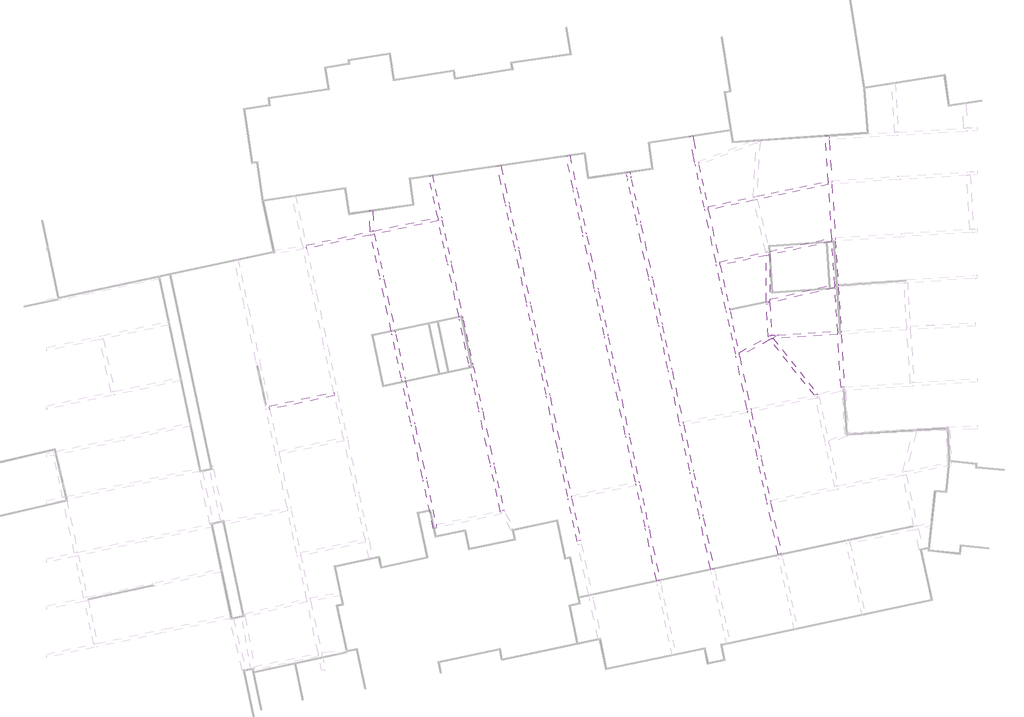
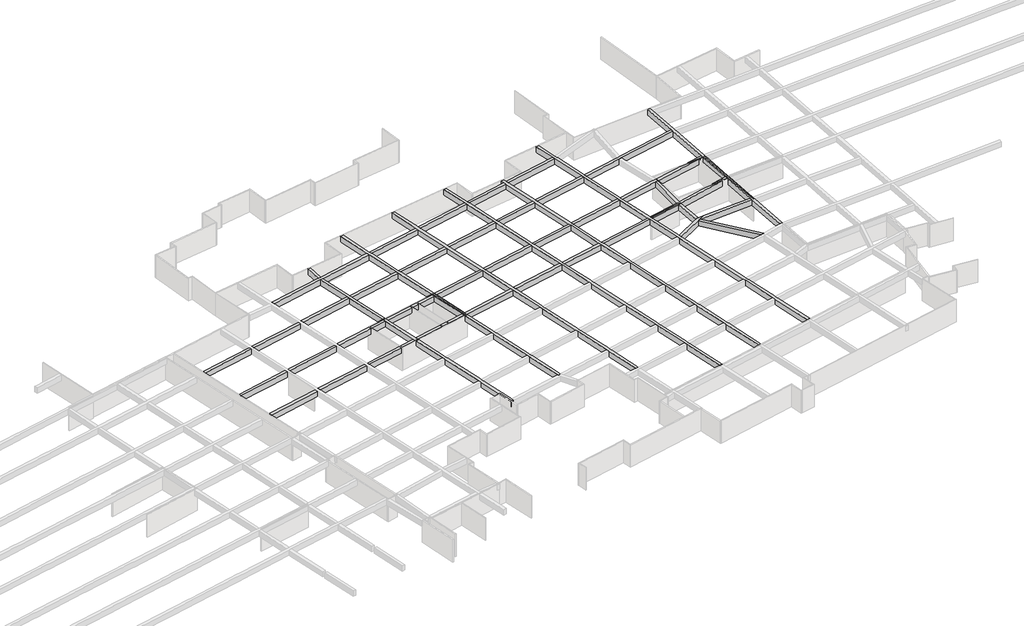
# One storey, part 10 of 14: 18 beams.
"""IFC4 building model written with IfcOpenShell, lengths in millimetres."""

from ifc_helpers import new_model, si_unit, frame, origin, place, context, project, spatial, polyline, outline, extrude, faceted_brep, element, save

model = new_model("IFC4")

# Units and contexts
model_context = context("Model", 3, world=origin())
ifc_project = project(units=[si_unit("LENGTHUNIT", "METRE", prefix="MILLI")], contexts=[model_context])

# Site, building, storey
site = spatial("IfcSite", under=ifc_project)
building = spatial("IfcBuilding", under=site)
storey = spatial("IfcBuildingStorey", under=building, Name="户型图", Elevation=0.0)

# Beams
placement = place(None, origin())
element("IfcBeam", 1, ObjectType="混凝土 - 矩形梁 : KL_beam", at=placement, inside=storey, context=model_context, shape_type="SweptSolid", body=[
    extrude(outline(polyline([(-247291.3597024, -139083.8420876), (-246891.9078885, -139062.9077051), (-246769.3406579, -141401.6297867), (-247165.4767913, -141485.8311212), (-247291.3597024, -139083.8420876)])), frame((0.0, 0.0, 2500.0), z_axis=(0.0, 0.0, 1.0), x_axis=(1.0, 0.0, 0.0)), (0.0, 0.0, 1.0), 800.0),
])
element("IfcBeam", 2, ObjectType="混凝土 - 矩形梁 : KL_beam", at=placement, inside=storey, context=model_context, shape_type="Brep", body=[
    faceted_brep([(-239502.5663622, -175696.1273321, 3300.0), (-239502.5663622, -175696.1273321, 2500.0), (-239585.7310386, -175304.8682918, 2500.0), (-240656.2680649, -170268.3875645, 2500.0), (-240739.4335016, -169877.124947, 2500.0), (-242007.8205291, -163909.833147, 2500.0), (-242090.9852054, -163518.5741067, 2500.0), (-243116.5813419, -158693.5236429, 2500.0), (-243199.7460182, -158302.2646026, 2500.0), (-244253.2667899, -153345.839059, 2500.0), (-244336.4314662, -152954.5800187, 2500.0), (-245612.0065383, -146953.4711277, 2500.0), (-245695.1712146, -146562.2120874, 2500.0), (-246707.9389128, -141797.5146808, 2500.0), (-246707.9389128, -141797.5146808, 3300.0), (-245695.1712146, -146562.2120874, 3300.0), (-245612.0065383, -146953.4711277, 3300.0), (-244336.4314662, -152954.5800187, 3300.0), (-244253.2667899, -153345.839059, 3300.0), (-243199.7460182, -158302.2646026, 3300.0), (-243116.5813419, -158693.5236429, 3300.0), (-242090.9852054, -163518.5741067, 3300.0), (-242007.8205291, -163909.833147, 3300.0), (-240739.4335016, -169877.124947, 3300.0), (-240656.2680649, -170268.3875645, 3300.0), (-239585.7310386, -175304.8682918, 3300.0), (-247099.1979531, -141880.6793572, 2500.0), (-247099.1979531, -141880.6793572, 3300.0), (-246086.4302549, -146645.3767637, 3300.0), (-246003.2655786, -147036.635804, 3300.0), (-244727.6905065, -153037.7446951, 3300.0), (-244644.5258302, -153429.0037354, 3300.0), (-243591.0050585, -158385.4292789, 3300.0), (-243507.8403822, -158776.6883192, 3300.0), (-242482.2442457, -163601.738783, 3300.0), (-242399.0795694, -163992.9978233, 3300.0), (-241130.3369189, -169961.9626978, 3300.0), (-241047.1714822, -170353.2253152, 3300.0), (-239893.8254025, -175779.2920084, 3300.0), (-246086.4302549, -146645.3767637, 2500.0), (-246003.2655786, -147036.635804, 2500.0), (-244727.6905065, -153037.7446951, 2500.0), (-244644.5258302, -153429.0037354, 2500.0), (-243591.0050585, -158385.4292789, 2500.0), (-243507.8403822, -158776.6883192, 2500.0), (-242482.2442457, -163601.738783, 2500.0), (-242399.0795694, -163992.9978233, 2500.0), (-241130.3369189, -169961.9626978, 2500.0), (-241047.1714822, -170353.2253152, 2500.0), (-239893.8254025, -175779.2920084, 2500.0)], [[[0, 1, 2, 3, 4, 5, 6, 7, 8, 9, 10, 11, 12, 13, 14, 15, 16, 17, 18, 19, 20, 21, 22, 23, 24, 25]], [[14, 13, 26, 27]], [[14, 27, 28, 29, 30, 31, 32, 33, 34, 35, 36, 37, 38, 0, 25, 24, 23, 22, 21, 20, 19, 18, 17, 16, 15]], [[27, 26, 39, 40, 41, 42, 43, 44, 45, 46, 47, 48, 49, 38, 37, 36, 35, 34, 33, 32, 31, 30, 29, 28]], [[26, 13, 12, 11, 10, 9, 8, 7, 6, 5, 4, 3, 2, 1, 49, 48, 47, 46, 45, 44, 43, 42, 41, 40, 39]], [[0, 38, 49, 1]]]),
])
element("IfcBeam", 3, ObjectType="混凝土 - 矩形梁 : KL_beam", at=placement, inside=storey, context=model_context, shape_type="Brep", body=[
    faceted_brep([(-240003.3061587, -134987.1905484, 3300.0), (-240003.3061587, -134987.1905484, 2500.0), (-240394.565199, -135070.3552247, 2500.0), (-240394.565199, -135070.3552247, 3300.0), (-232154.5574648, -173836.5437133, 3300.0), (-231776.7079802, -173690.2920379, 3300.0), (-231785.9170748, -173646.966654, 3300.0), (-232863.5435036, -168577.1329101, 3300.0), (-232946.7089403, -168185.8702927, 3300.0), (-234208.0065653, -162251.9315092, 3300.0), (-234291.1712416, -161860.6724689, 3300.0), (-235316.7673781, -157035.6220051, 3300.0), (-235399.9320544, -156644.3629648, 3300.0), (-236453.4528261, -151687.9374212, 3300.0), (-236536.6175025, -151296.6783809, 3300.0), (-237812.1925745, -145295.5694899, 3300.0), (-237895.3572509, -144904.3104496, 3300.0), (-238908.124949, -140139.613043, 3300.0), (-238991.2896253, -139748.3540027, 3300.0), (-239382.5486656, -139831.5186791, 3300.0), (-239299.3839893, -140222.7777194, 3300.0), (-238286.6162912, -144987.4751259, 3300.0), (-238203.4516148, -145378.7341662, 3300.0), (-236927.8765428, -151379.8430573, 3300.0), (-236844.7118664, -151771.1020976, 3300.0), (-235791.1910947, -156727.5276411, 3300.0), (-235708.0264184, -157118.7866814, 3300.0), (-234682.4302819, -161943.8371452, 3300.0), (-234599.2656056, -162335.0961855, 3300.0), (-233337.6123577, -168270.7080435, 3300.0), (-233254.446921, -168661.9706609, 3300.0), (-232177.1761151, -173730.1313303, 3300.0), (-232154.5574648, -173836.5437133, 2500.0), (-239382.5486656, -139831.5186791, 2500.0), (-239299.3839893, -140222.7777194, 2500.0), (-238286.6162912, -144987.4751259, 2500.0), (-238203.4516148, -145378.7341662, 2500.0), (-236927.8765428, -151379.8430573, 2500.0), (-236844.7118664, -151771.1020976, 2500.0), (-235791.1910947, -156727.5276411, 2500.0), (-235708.0264184, -157118.7866814, 2500.0), (-234682.4302819, -161943.8371452, 2500.0), (-234599.2656056, -162335.0961855, 2500.0), (-233337.6123577, -168270.7080435, 2500.0), (-233254.446921, -168661.9706609, 2500.0), (-232177.1761151, -173730.1313303, 2500.0), (-231776.7079802, -173690.2920379, 2500.0), (-238991.2896253, -139748.3540027, 2500.0), (-238908.124949, -140139.613043, 2500.0), (-237895.3572509, -144904.3104496, 2500.0), (-237812.1925745, -145295.5694899, 2500.0), (-236536.6175025, -151296.6783809, 2500.0), (-236453.4528261, -151687.9374212, 2500.0), (-235399.9320544, -156644.3629648, 2500.0), (-235316.7673781, -157035.6220051, 2500.0), (-234291.1712416, -161860.6724689, 2500.0), (-234208.0065653, -162251.9315092, 2500.0), (-232946.7089403, -168185.8702927, 2500.0), (-232863.5435036, -168577.1329101, 2500.0), (-231785.9170748, -173646.966654, 2500.0)], [[[0, 1, 2, 3]], [[4, 5, 6, 7, 8, 9, 10, 11, 12, 13, 14, 15, 16, 17, 18, 0, 3, 19, 20, 21, 22, 23, 24, 25, 26, 27, 28, 29, 30, 31]], [[32, 4, 31, 30, 29, 28, 27, 26, 25, 24, 23, 22, 21, 20, 19, 3, 2, 33, 34, 35, 36, 37, 38, 39, 40, 41, 42, 43, 44, 45]], [[46, 32, 45, 44, 43, 42, 41, 40, 39, 38, 37, 36, 35, 34, 33, 2, 1, 47, 48, 49, 50, 51, 52, 53, 54, 55, 56, 57, 58, 59]], [[5, 46, 59, 58, 57, 56, 55, 54, 53, 52, 51, 50, 49, 48, 47, 1, 0, 18, 17, 16, 15, 14, 13, 12, 11, 10, 9, 8, 7, 6]], [[5, 4, 32, 46]]]),
])
element("IfcBeam", 4, ObjectType="混凝土 - 矩形梁 : KL_beam", at=placement, inside=storey, context=model_context, shape_type="Brep", body=[
    faceted_brep([(-232107.9736676, -133827.7635984, 3300.0), (-232107.9736676, -133827.7635984, 2500.0), (-232499.2327078, -133910.9282747, 2500.0), (-232499.2327078, -133910.9282747, 3300.0), (-231592.7191403, -138175.7392992, 3300.0), (-231509.554464, -138566.9983395, 3300.0), (-230496.7867659, -143331.695746, 3300.0), (-230413.6220895, -143722.9547863, 3300.0), (-229138.0470174, -149724.0636774, 3300.0), (-229054.8823411, -150115.3227177, 3300.0), (-228001.3615694, -155071.7482612, 3300.0), (-227918.1968931, -155463.0073015, 3300.0), (-226892.6007566, -160288.0577653, 3300.0), (-226809.4360803, -160679.3168056, 3300.0), (-225554.8631598, -166581.6183418, 3300.0), (-225471.6977231, -166972.8809592, 3300.0), (-224387.3465898, -172074.3519504, 3300.0), (-224304.1819135, -172465.6109907, 3300.0), (-223290.3781842, -177235.1825406, 3300.0), (-222899.1191439, -177152.0178643, 3300.0), (-223912.9228732, -172382.4463144, 3300.0), (-223996.0875495, -171991.1872741, 3300.0), (-225080.7943058, -166888.0432085, 3300.0), (-225163.9597425, -166496.7805911, 3300.0), (-226418.17704, -160596.1521293, 3300.0), (-226501.3417163, -160204.893089, 3300.0), (-227526.9378528, -155379.8426252, 3300.0), (-227610.1025291, -154988.5835849, 3300.0), (-228663.6233008, -150032.1580413, 3300.0), (-228746.7879771, -149640.899001, 3300.0), (-230022.3630492, -143639.79011, 3300.0), (-230105.5277256, -143248.5310697, 3300.0), (-231118.2954237, -138483.8336631, 3300.0), (-231201.4601, -138092.5746229, 3300.0), (-231592.7191403, -138175.7392992, 2500.0), (-231509.554464, -138566.9983395, 2500.0), (-230496.7867659, -143331.695746, 2500.0), (-230413.6220895, -143722.9547863, 2500.0), (-229138.0470174, -149724.0636774, 2500.0), (-229054.8823411, -150115.3227177, 2500.0), (-228001.3615694, -155071.7482612, 2500.0), (-227918.1968931, -155463.0073015, 2500.0), (-226892.6007566, -160288.0577653, 2500.0), (-226809.4360803, -160679.3168056, 2500.0), (-225554.8631598, -166581.6183418, 2500.0), (-225471.6977231, -166972.8809592, 2500.0), (-224387.3465898, -172074.3519504, 2500.0), (-224304.1819135, -172465.6109907, 2500.0), (-223290.3781842, -177235.1825406, 2500.0), (-231201.4601, -138092.5746229, 2500.0), (-231118.2954237, -138483.8336631, 2500.0), (-230105.5277256, -143248.5310697, 2500.0), (-230022.3630492, -143639.79011, 2500.0), (-228746.7879771, -149640.899001, 2500.0), (-228663.6233008, -150032.1580413, 2500.0), (-227610.1025291, -154988.5835849, 2500.0), (-227526.9378528, -155379.8426252, 2500.0), (-226501.3417163, -160204.893089, 2500.0), (-226418.17704, -160596.1521293, 2500.0), (-225163.9597425, -166496.7805911, 2500.0), (-225080.7943058, -166888.0432085, 2500.0), (-223996.0875495, -171991.1872741, 2500.0), (-223912.9228732, -172382.4463144, 2500.0), (-222899.1191439, -177152.0178643, 2500.0)], [[[0, 1, 2, 3]], [[0, 3, 4, 5, 6, 7, 8, 9, 10, 11, 12, 13, 14, 15, 16, 17, 18, 19, 20, 21, 22, 23, 24, 25, 26, 27, 28, 29, 30, 31, 32, 33]], [[3, 2, 34, 35, 36, 37, 38, 39, 40, 41, 42, 43, 44, 45, 46, 47, 48, 18, 17, 16, 15, 14, 13, 12, 11, 10, 9, 8, 7, 6, 5, 4]], [[2, 1, 49, 50, 51, 52, 53, 54, 55, 56, 57, 58, 59, 60, 61, 62, 63, 48, 47, 46, 45, 44, 43, 42, 41, 40, 39, 38, 37, 36, 35, 34]], [[1, 0, 33, 32, 31, 30, 29, 28, 27, 26, 25, 24, 23, 22, 21, 20, 19, 63, 62, 61, 60, 59, 58, 57, 56, 55, 54, 53, 52, 51, 50, 49]], [[19, 18, 48, 63]]]),
])
element("IfcBeam", 5, ObjectType="混凝土 - 矩形梁 : KL_beam", at=placement, inside=storey, context=model_context, shape_type="Brep", body=[
    faceted_brep([(-224568.0292654, -132746.4320366, 3300.0), (-224176.7702251, -132663.2673603, 3300.0), (-224176.7702251, -132663.2673603, 2500.0), (-224568.0292654, -132746.4320366, 2500.0), (-223767.5383344, -136512.4457726, 3300.0), (-223684.3736581, -136903.7048129, 3300.0), (-222671.60596, -141668.4022195, 3300.0), (-222588.4412837, -142059.6612598, 3300.0), (-221312.8662116, -148060.7701508, 3300.0), (-221229.7015352, -148452.0291911, 3300.0), (-220176.1807635, -153408.4547347, 3300.0), (-220093.0160872, -153799.713775, 3300.0), (-219067.4199507, -158624.7642388, 3300.0), (-218984.2552744, -159016.023279, 3300.0), (-217736.7948129, -164884.8633268, 3300.0), (-217653.6293762, -165276.1259443, 3300.0), (-216562.1657839, -170411.0584239, 3300.0), (-216479.0011076, -170802.3174642, 3300.0), (-215465.1973783, -175571.8890141, 3300.0), (-215382.032702, -175963.1480544, 3300.0), (-214134.7118605, -181831.3312414, 3300.0), (-213743.4528202, -181748.166565, 3300.0), (-214990.7736617, -175879.9833781, 3300.0), (-215073.938338, -175488.7243378, 3300.0), (-216087.7420673, -170719.1527879, 3300.0), (-216170.9067436, -170327.8937476, 3300.0), (-217262.7259588, -165191.2881935, 3300.0), (-217345.8913955, -164800.0255761, 3300.0), (-218592.9962341, -158932.8586027, 3300.0), (-218676.1609104, -158541.5995624, 3300.0), (-219701.7570469, -153716.5490987, 3300.0), (-219784.9217232, -153325.2900584, 3300.0), (-220838.4424949, -148368.8645148, 3300.0), (-220921.6071713, -147977.6054745, 3300.0), (-222197.1822434, -141976.4965835, 3300.0), (-222280.3469197, -141585.2375432, 3300.0), (-223293.1146178, -136820.5401366, 3300.0), (-223376.2792942, -136429.2810963, 3300.0), (-213743.4528202, -181748.166565, 2500.0), (-214990.7736617, -175879.9833781, 2500.0), (-215073.938338, -175488.7243378, 2500.0), (-216087.7420673, -170719.1527879, 2500.0), (-216170.9067436, -170327.8937476, 2500.0), (-217262.7259588, -165191.2881935, 2500.0), (-217345.8913955, -164800.0255761, 2500.0), (-218592.9962341, -158932.8586027, 2500.0), (-218676.1609104, -158541.5995624, 2500.0), (-219701.7570469, -153716.5490987, 2500.0), (-219784.9217232, -153325.2900584, 2500.0), (-220838.4424949, -148368.8645148, 2500.0), (-220921.6071713, -147977.6054745, 2500.0), (-222197.1822434, -141976.4965835, 2500.0), (-222280.3469197, -141585.2375432, 2500.0), (-223293.1146178, -136820.5401366, 2500.0), (-223376.2792942, -136429.2810963, 2500.0), (-214134.7118605, -181831.3312414, 2500.0), (-215382.032702, -175963.1480544, 2500.0), (-215465.1973783, -175571.8890141, 2500.0), (-216479.0011076, -170802.3174642, 2500.0), (-216562.1657839, -170411.0584239, 2500.0), (-217653.6293762, -165276.1259443, 2500.0), (-217736.7948129, -164884.8633268, 2500.0), (-218984.2552744, -159016.023279, 2500.0), (-219067.4199507, -158624.7642388, 2500.0), (-220093.0160872, -153799.713775, 2500.0), (-220176.1807635, -153408.4547347, 2500.0), (-221229.7015352, -148452.0291911, 2500.0), (-221312.8662116, -148060.7701508, 2500.0), (-222588.4412837, -142059.6612598, 2500.0), (-222671.60596, -141668.4022195, 2500.0), (-223684.3736581, -136903.7048129, 2500.0), (-223767.5383344, -136512.4457726, 2500.0)], [[[0, 1, 2, 3]], [[1, 0, 4, 5, 6, 7, 8, 9, 10, 11, 12, 13, 14, 15, 16, 17, 18, 19, 20, 21, 22, 23, 24, 25, 26, 27, 28, 29, 30, 31, 32, 33, 34, 35, 36, 37]], [[2, 1, 37, 36, 35, 34, 33, 32, 31, 30, 29, 28, 27, 26, 25, 24, 23, 22, 21, 38, 39, 40, 41, 42, 43, 44, 45, 46, 47, 48, 49, 50, 51, 52, 53, 54]], [[3, 2, 54, 53, 52, 51, 50, 49, 48, 47, 46, 45, 44, 43, 42, 41, 40, 39, 38, 55, 56, 57, 58, 59, 60, 61, 62, 63, 64, 65, 66, 67, 68, 69, 70, 71]], [[0, 3, 71, 70, 69, 68, 67, 66, 65, 64, 63, 62, 61, 60, 59, 58, 57, 56, 55, 20, 19, 18, 17, 16, 15, 14, 13, 12, 11, 10, 9, 8, 7, 6, 5, 4]], [[20, 55, 38, 21]]]),
])
element("IfcBeam", 6, ObjectType="混凝土 - 矩形梁 : KL_beam", at=placement, inside=storey, context=model_context, shape_type="Brep", body=[
    faceted_brep([(-217241.693878, -134575.5020687, 3300.0), (-217241.693878, -134575.5020687, 2500.0), (-217632.9529183, -134658.666745, 2500.0), (-217632.9529183, -134658.666745, 3300.0), (-207888.3079023, -180503.6170932, 3300.0), (-207497.048862, -180420.4524169, 3300.0), (-208744.3697035, -174552.2692299, 3300.0), (-208827.5343798, -174161.0101896, 3300.0), (-209841.3381091, -169391.4386397, 3300.0), (-209924.5027854, -169000.1795994, 3300.0), (-211021.0898908, -163841.1428861, 3300.0), (-211104.2672354, -163449.824246, 3300.0), (-212346.5922759, -157605.1444546, 3300.0), (-212429.7569523, -157213.8854143, 3300.0), (-213455.3530887, -152388.8349505, 3300.0), (-213538.5177651, -151997.5759102, 3300.0), (-214592.0385368, -147041.1503666, 3300.0), (-214675.2032131, -146649.8913263, 3300.0), (-215950.7782852, -140648.7824353, 3300.0), (-216033.9429615, -140257.523395, 3300.0), (-217046.7106596, -135492.8259885, 3300.0), (-217129.875336, -135101.5669482, 3300.0), (-217521.1343763, -135184.7316245, 3300.0), (-217437.9696999, -135575.9906648, 3300.0), (-216425.2020018, -140340.6880713, 3300.0), (-216342.0373255, -140731.9471116, 3300.0), (-215066.4622534, -146733.0560027, 3300.0), (-214983.2975771, -147124.315043, 3300.0), (-213929.7768053, -152080.7405865, 3300.0), (-213846.612129, -152471.9996268, 3300.0), (-212821.0159926, -157297.0500906, 3300.0), (-212737.8513162, -157688.3091309, 3300.0), (-211496.0683326, -163530.4387449, 3300.0), (-211412.902896, -163921.7013623, 3300.0), (-210315.7618257, -169083.3442757, 3300.0), (-210232.5971494, -169474.603316, 3300.0), (-209218.7934201, -174244.1748659, 3300.0), (-209135.6287438, -174635.4339062, 3300.0), (-207888.3079023, -180503.6170932, 2500.0), (-217521.1343763, -135184.7316245, 2500.0), (-217437.9696999, -135575.9906648, 2500.0), (-216425.2020018, -140340.6880713, 2500.0), (-216342.0373255, -140731.9471116, 2500.0), (-215066.4622534, -146733.0560027, 2500.0), (-214983.2975771, -147124.315043, 2500.0), (-213929.7768053, -152080.7405865, 2500.0), (-213846.612129, -152471.9996268, 2500.0), (-212821.0159926, -157297.0500906, 2500.0), (-212737.8513162, -157688.3091309, 2500.0), (-211496.0683326, -163530.4387449, 2500.0), (-211412.902896, -163921.7013623, 2500.0), (-210315.7618257, -169083.3442757, 2500.0), (-210232.5971494, -169474.603316, 2500.0), (-209218.7934201, -174244.1748659, 2500.0), (-209135.6287438, -174635.4339062, 2500.0), (-207497.048862, -180420.4524169, 2500.0), (-217129.875336, -135101.5669482, 2500.0), (-217046.7106596, -135492.8259885, 2500.0), (-216033.9429615, -140257.523395, 2500.0), (-215950.7782852, -140648.7824353, 2500.0), (-214675.2032131, -146649.8913263, 2500.0), (-214592.0385368, -147041.1503666, 2500.0), (-213538.5177651, -151997.5759102, 2500.0), (-213455.3530887, -152388.8349505, 2500.0), (-212429.7569523, -157213.8854143, 2500.0), (-212346.5922759, -157605.1444546, 2500.0), (-211104.2672354, -163449.824246, 2500.0), (-211021.0898908, -163841.1428861, 2500.0), (-209924.5027854, -169000.1795994, 2500.0), (-209841.3381091, -169391.4386397, 2500.0), (-208827.5343798, -174161.0101896, 2500.0), (-208744.3697035, -174552.2692299, 2500.0)], [[[0, 1, 2, 3]], [[4, 5, 6, 7, 8, 9, 10, 11, 12, 13, 14, 15, 16, 17, 18, 19, 20, 21, 0, 3, 22, 23, 24, 25, 26, 27, 28, 29, 30, 31, 32, 33, 34, 35, 36, 37]], [[38, 4, 37, 36, 35, 34, 33, 32, 31, 30, 29, 28, 27, 26, 25, 24, 23, 22, 3, 2, 39, 40, 41, 42, 43, 44, 45, 46, 47, 48, 49, 50, 51, 52, 53, 54]], [[55, 38, 54, 53, 52, 51, 50, 49, 48, 47, 46, 45, 44, 43, 42, 41, 40, 39, 2, 1, 56, 57, 58, 59, 60, 61, 62, 63, 64, 65, 66, 67, 68, 69, 70, 71]], [[5, 55, 71, 70, 69, 68, 67, 66, 65, 64, 63, 62, 61, 60, 59, 58, 57, 56, 1, 0, 21, 20, 19, 18, 17, 16, 15, 14, 13, 12, 11, 10, 9, 8, 7, 6]], [[5, 4, 38, 55]]]),
])
element("IfcBeam", 7, ObjectType="混凝土 - 矩形梁 : KL_beam", at=placement, inside=storey, context=model_context, shape_type="Brep", body=[
    faceted_brep([(-210361.4643641, -130516.7008137, 3300.0), (-209970.2053238, -130433.5361374, 3300.0), (-209970.2053238, -130433.5361374, 2500.0), (-210361.4643641, -130516.7008137, 2500.0), (-209721.6277704, -133526.8953176, 3300.0), (-209638.463094, -133918.1543579, 3300.0), (-208625.6953959, -138682.8517645, 3300.0), (-208542.5307196, -139074.1108048, 3300.0), (-207266.9556475, -145075.2196958, 3300.0), (-207183.7909711, -145466.4787361, 3300.0), (-206130.2701994, -150422.9042797, 3300.0), (-206047.1055231, -150814.16332, 3300.0), (-205021.5093866, -155639.2137837, 3300.0), (-204938.3447103, -156030.472824, 3300.0), (-203668.5336742, -162004.4640578, 3300.0), (-203585.3563296, -162395.7826978, 3300.0), (-202516.2552198, -167425.5079689, 3300.0), (-202433.0905435, -167816.7670092, 3300.0), (-201419.2868142, -172586.3385591, 3300.0), (-201336.1221379, -172977.5975994, 3300.0), (-200110.5246312, -178743.5805315, 3300.0), (-199719.2655909, -178660.4158551, 3300.0), (-200944.8630976, -172894.432923, 3300.0), (-201028.0277739, -172503.1738827, 3300.0), (-202041.8315032, -167733.6023328, 3300.0), (-202124.9961795, -167342.3432925, 3300.0), (-203193.377801, -162316.0029476, 3300.0), (-203276.5424774, -161924.7439073, 3300.0), (-204557.8986965, -155896.4368576, 3300.0), (-204644.863313, -155487.3005045, 3300.0), (-205655.8464828, -150730.9986436, 3300.0), (-205739.0111591, -150339.7396033, 3300.0), (-206792.5319309, -145383.3140598, 3300.0), (-206875.6966072, -144992.0550195, 3300.0), (-208151.2716793, -138990.9461284, 3300.0), (-208234.4363556, -138599.6870881, 3300.0), (-209253.2346635, -133806.6178935, 3300.0), (-209337.422307, -133410.5461707, 3300.0), (-199719.2655909, -178660.4158551, 2500.0), (-200944.8630976, -172894.432923, 2500.0), (-201028.0277739, -172503.1738827, 2500.0), (-202041.8315032, -167733.6023328, 2500.0), (-202124.9961795, -167342.3432925, 2500.0), (-203193.377801, -162316.0029476, 2500.0), (-203276.5424774, -161924.7439073, 2500.0), (-204557.8986965, -155896.4368576, 2500.0), (-204644.863313, -155487.3005045, 2500.0), (-205655.8464828, -150730.9986436, 2500.0), (-205739.0111591, -150339.7396033, 2500.0), (-206792.5319309, -145383.3140598, 2500.0), (-206875.6966072, -144992.0550195, 2500.0), (-208151.2716793, -138990.9461284, 2500.0), (-208234.4363556, -138599.6870881, 2500.0), (-209253.2346635, -133806.6178935, 2500.0), (-209337.422307, -133410.5461707, 2500.0), (-200110.5246312, -178743.5805315, 2500.0), (-201336.1221379, -172977.5975994, 2500.0), (-201419.2868142, -172586.3385591, 2500.0), (-202433.0905435, -167816.7670092, 2500.0), (-202516.2552198, -167425.5079689, 2500.0), (-203585.3563296, -162395.7826978, 2500.0), (-203668.5336742, -162004.4640578, 2500.0), (-204938.3447103, -156030.472824, 2500.0), (-205021.5093866, -155639.2137837, 2500.0), (-206047.1055231, -150814.16332, 2500.0), (-206130.2701994, -150422.9042797, 2500.0), (-207183.7909711, -145466.4787361, 2500.0), (-207266.9556475, -145075.2196958, 2500.0), (-208542.5307196, -139074.1108048, 2500.0), (-208625.6953959, -138682.8517645, 2500.0), (-209638.463094, -133918.1543579, 2500.0), (-209721.6277704, -133526.8953176, 2500.0)], [[[0, 1, 2, 3]], [[1, 0, 4, 5, 6, 7, 8, 9, 10, 11, 12, 13, 14, 15, 16, 17, 18, 19, 20, 21, 22, 23, 24, 25, 26, 27, 28, 29, 30, 31, 32, 33, 34, 35, 36, 37]], [[2, 1, 37, 36, 35, 34, 33, 32, 31, 30, 29, 28, 27, 26, 25, 24, 23, 22, 21, 38, 39, 40, 41, 42, 43, 44, 45, 46, 47, 48, 49, 50, 51, 52, 53, 54]], [[3, 2, 54, 53, 52, 51, 50, 49, 48, 47, 46, 45, 44, 43, 42, 41, 40, 39, 38, 55, 56, 57, 58, 59, 60, 61, 62, 63, 64, 65, 66, 67, 68, 69, 70, 71]], [[0, 3, 71, 70, 69, 68, 67, 66, 65, 64, 63, 62, 61, 60, 59, 58, 57, 56, 55, 20, 19, 18, 17, 16, 15, 14, 13, 12, 11, 10, 9, 8, 7, 6, 5, 4]], [[20, 55, 38, 21]]]),
])
element("IfcBeam", 8, ObjectType="混凝土 - 矩形梁 : KL_beam", at=placement, inside=storey, context=model_context, shape_type="Brep", body=[
    faceted_brep([(-201469.3690271, -149705.3712489, 3300.0), (-201069.3690271, -149705.3712489, 3300.0), (-201069.3690271, -149294.7612479, 3300.0), (-201069.3690271, -144166.8182311, 3300.0), (-201469.3690271, -144251.8408557, 3300.0), (-201469.3690271, -149432.1991522, 3300.0), (-201469.3690271, -149705.3712489, 2500.0), (-201469.3690271, -144251.8408557, 2500.0), (-201469.3690271, -149432.1991522, 2500.0), (-201069.3690271, -149705.3712489, 2500.0), (-201069.3690271, -144166.8182311, 2500.0), (-201069.3690271, -149294.7612479, 2500.0)], [[[0, 1, 2, 3, 4, 5]], [[6, 0, 5, 4, 7, 8]], [[9, 6, 8, 7, 10, 11]], [[1, 9, 11, 10, 3, 2]], [[1, 0, 6, 9]], [[3, 10, 7, 4]]]),
])
element("IfcBeam", 9, ObjectType="混凝土 - 矩形梁 : KL_beam", at=placement, inside=storey, context=model_context, shape_type="Brep", body=[
    faceted_brep([(-269185.8351032, -151555.3068349, 3300.0), (-269185.8351032, -151555.3068349, 2500.0), (-269102.6704268, -151946.5658752, 2500.0), (-269102.6704268, -151946.5658752, 3300.0), (-261736.5979738, -149971.9226036, 3300.0), (-261653.4332975, -150363.1816439, 3300.0), (-261653.4332975, -150363.1816439, 2500.0), (-261736.5979738, -149971.9226036, 2500.0)], [[[0, 1, 2, 3]], [[4, 5, 6, 7]], [[0, 3, 5, 4]], [[3, 2, 6, 5]], [[2, 1, 7, 6]], [[1, 0, 4, 7]]]),
    faceted_brep([(-208234.4363556, -138599.6870881, 3300.0), (-208151.2716793, -138990.9461284, 3300.0), (-202914.7402599, -137877.8870148, 3300.0), (-202523.4216199, -137794.7096702, 3300.0), (-194295.6524967, -136045.8433552, 3300.0), (-194320.579007, -135642.2054105, 3300.0), (-202549.7970747, -137391.3797083, 3300.0), (-202955.2359711, -137477.558406, 3300.0), (-208151.2716793, -138990.9461284, 2500.0), (-202914.7402599, -137877.8870148, 2500.0), (-202523.4216199, -137794.7096702, 2500.0), (-194295.6524967, -136045.8433552, 2500.0), (-208234.4363556, -138599.6870881, 2500.0), (-202955.2359711, -137477.558406, 2500.0), (-202549.7970747, -137391.3797083, 2500.0), (-194320.579007, -135642.2054105, 2500.0)], [[[0, 1, 2, 3, 4, 5, 6, 7]], [[1, 8, 9, 10, 11, 4, 3, 2]], [[8, 12, 13, 14, 15, 11, 10, 9]], [[12, 0, 7, 6, 5, 15, 14, 13]], [[1, 0, 12, 8]], [[5, 4, 11, 15]]]),
    faceted_brep([(-261262.1742572, -150280.0169676, 3300.0), (-261345.3389335, -149888.7579273, 3300.0), (-261345.3389335, -149888.7579273, 2500.0), (-261262.1742572, -150280.0169676, 2500.0), (-253874.8161124, -148300.8492826, 3300.0), (-253791.6514361, -148692.1083228, 3300.0), (-253791.6514361, -148692.1083228, 2500.0), (-253874.8161124, -148300.8492826, 2500.0)], [[[0, 1, 2, 3]], [[4, 5, 6, 7]], [[1, 0, 5, 4]], [[0, 3, 6, 5]], [[3, 2, 7, 6]], [[2, 1, 4, 7]]]),
    faceted_brep([(-253400.3923958, -148608.9436465, 3300.0), (-253483.5570721, -148217.6846062, 3300.0), (-253483.5570721, -148217.6846062, 2500.0), (-253400.3923958, -148608.9436465, 2500.0), (-246086.4302549, -146645.3767637, 3300.0), (-246003.2655786, -147036.635804, 3300.0), (-246003.2655786, -147036.635804, 2500.0), (-246086.4302549, -146645.3767637, 2500.0)], [[[0, 1, 2, 3]], [[4, 5, 6, 7]], [[1, 0, 5, 4]], [[0, 3, 6, 5]], [[3, 2, 7, 6]], [[2, 1, 4, 7]]]),
    faceted_brep([(-245612.0065383, -146953.4711277, 3300.0), (-245695.1712146, -146562.2120874, 3300.0), (-245695.1712146, -146562.2120874, 2500.0), (-245612.0065383, -146953.4711277, 2500.0), (-238286.6162912, -144987.4751259, 3300.0), (-238203.4516148, -145378.7341662, 3300.0), (-238203.4516148, -145378.7341662, 2500.0), (-238286.6162912, -144987.4751259, 2500.0)], [[[0, 1, 2, 3]], [[4, 5, 6, 7]], [[1, 0, 5, 4]], [[0, 3, 6, 5]], [[3, 2, 7, 6]], [[2, 1, 4, 7]]]),
    faceted_brep([(-237812.1925745, -145295.5694899, 3300.0), (-237895.3572509, -144904.3104496, 3300.0), (-237895.3572509, -144904.3104496, 2500.0), (-237812.1925745, -145295.5694899, 2500.0), (-230496.7867659, -143331.695746, 3300.0), (-230413.6220895, -143722.9547863, 3300.0), (-230413.6220895, -143722.9547863, 2500.0), (-230496.7867659, -143331.695746, 2500.0)], [[[0, 1, 2, 3]], [[4, 5, 6, 7]], [[1, 0, 5, 4]], [[0, 3, 6, 5]], [[3, 2, 7, 6]], [[2, 1, 4, 7]]]),
    faceted_brep([(-230022.3630492, -143639.79011, 3300.0), (-230105.5277256, -143248.5310697, 3300.0), (-230105.5277256, -143248.5310697, 2500.0), (-230022.3630492, -143639.79011, 2500.0), (-222671.60596, -141668.4022195, 3300.0), (-222588.4412837, -142059.6612598, 3300.0), (-222588.4412837, -142059.6612598, 2500.0), (-222671.60596, -141668.4022195, 2500.0)], [[[0, 1, 2, 3]], [[4, 5, 6, 7]], [[1, 0, 5, 4]], [[0, 3, 6, 5]], [[3, 2, 7, 6]], [[2, 1, 4, 7]]]),
    faceted_brep([(-222197.1822434, -141976.4965835, 3300.0), (-222280.3469197, -141585.2375432, 3300.0), (-222280.3469197, -141585.2375432, 2500.0), (-222197.1822434, -141976.4965835, 2500.0), (-216425.2020018, -140340.6880713, 3300.0), (-216342.0373255, -140731.9471116, 3300.0), (-216342.0373255, -140731.9471116, 2500.0), (-216425.2020018, -140340.6880713, 2500.0)], [[[0, 1, 2, 3]], [[4, 5, 6, 7]], [[1, 0, 5, 4]], [[0, 3, 6, 5]], [[3, 2, 7, 6]], [[2, 1, 4, 7]]]),
    faceted_brep([(-215950.7782852, -140648.7824353, 3300.0), (-216033.9429615, -140257.523395, 3300.0), (-216033.9429615, -140257.523395, 2500.0), (-215950.7782852, -140648.7824353, 2500.0), (-208625.6953959, -138682.8517645, 3300.0), (-208542.5307196, -139074.1108048, 3300.0), (-208542.5307196, -139074.1108048, 2500.0), (-208625.6953959, -138682.8517645, 2500.0)], [[[0, 1, 2, 3]], [[4, 5, 6, 7]], [[1, 0, 5, 4]], [[0, 3, 6, 5]], [[3, 2, 7, 6]], [[2, 1, 4, 7]]]),
])
element("IfcBeam", 10, ObjectType="混凝土 - 矩形梁 : KL_beam", at=placement, inside=storey, context=model_context, shape_type="Brep", body=[
    faceted_brep([(-254579.4894466, -143061.7281594, 3300.0), (-254496.3247703, -143452.9871997, 3300.0), (-247099.1979531, -141880.6793572, 3300.0), (-246707.9389128, -141797.5146808, 3300.0), (-239299.3839893, -140222.7777194, 3300.0), (-239382.5486656, -139831.5186791, 3300.0), (-246769.3406579, -141401.6297867, 3300.0), (-247165.4767913, -141485.8311212, 3300.0), (-254496.3247703, -143452.9871997, 2500.0), (-247099.1979531, -141880.6793572, 2500.0), (-246707.9389128, -141797.5146808, 2500.0), (-239299.3839893, -140222.7777194, 2500.0), (-254579.4894466, -143061.7281594, 2500.0), (-247165.4767913, -141485.8311212, 2500.0), (-246769.3406579, -141401.6297867, 2500.0), (-239382.5486656, -139831.5186791, 2500.0)], [[[0, 1, 2, 3, 4, 5, 6, 7]], [[1, 8, 9, 10, 11, 4, 3, 2]], [[8, 12, 13, 14, 15, 11, 10, 9]], [[12, 0, 7, 6, 5, 15, 14, 13]], [[1, 0, 12, 8]], [[5, 4, 11, 15]]]),
    faceted_brep([(-209721.6277704, -133526.8953176, 3300.0), (-209638.463094, -133918.1543579, 3300.0), (-209638.463094, -133918.1543579, 2500.0), (-209721.6277704, -133526.8953176, 2500.0), (-217129.875336, -135101.5669482, 3300.0), (-217046.7106596, -135492.8259885, 3300.0), (-217046.7106596, -135492.8259885, 2500.0), (-217129.875336, -135101.5669482, 2500.0)], [[[0, 1, 2, 3]], [[1, 0, 4, 5]], [[2, 1, 5, 6]], [[3, 2, 6, 7]], [[0, 3, 7, 4]], [[5, 4, 7, 6]]]),
    faceted_brep([(-238908.124949, -140139.613043, 3300.0), (-238991.2896253, -139748.3540027, 3300.0), (-238991.2896253, -139748.3540027, 2500.0), (-238908.124949, -140139.613043, 2500.0), (-231592.7191403, -138175.7392992, 3300.0), (-231509.554464, -138566.9983395, 3300.0), (-231509.554464, -138566.9983395, 2500.0), (-231592.7191403, -138175.7392992, 2500.0)], [[[0, 1, 2, 3]], [[4, 5, 6, 7]], [[1, 0, 5, 4]], [[0, 3, 6, 5]], [[3, 2, 7, 6]], [[2, 1, 4, 7]]]),
    faceted_brep([(-231201.4601, -138092.5746229, 3300.0), (-231118.2954237, -138483.8336631, 3300.0), (-223684.3736581, -136903.7048129, 3300.0), (-223767.5383344, -136512.4457726, 3300.0), (-231118.2954237, -138483.8336631, 2500.0), (-223684.3736581, -136903.7048129, 2500.0), (-231201.4601, -138092.5746229, 2500.0), (-223767.5383344, -136512.4457726, 2500.0)], [[[0, 1, 2, 3]], [[1, 4, 5, 2]], [[4, 6, 7, 5]], [[6, 0, 3, 7]], [[1, 0, 6, 4]], [[3, 2, 5, 7]]]),
    faceted_brep([(-223293.1146178, -136820.5401366, 3300.0), (-223376.2792942, -136429.2810963, 3300.0), (-223376.2792942, -136429.2810963, 2500.0), (-223293.1146178, -136820.5401366, 2500.0), (-217521.1343763, -135184.7316245, 3300.0), (-217437.9696999, -135575.9906648, 3300.0), (-217437.9696999, -135575.9906648, 2500.0), (-217521.1343763, -135184.7316245, 2500.0)], [[[0, 1, 2, 3]], [[4, 5, 6, 7]], [[1, 0, 5, 4]], [[0, 3, 6, 5]], [[3, 2, 7, 6]], [[2, 1, 4, 7]]]),
])
element("IfcBeam", 11, ObjectType="混凝土 - 矩形梁 : KL_beam", at=placement, inside=storey, context=model_context, shape_type="Brep", body=[
    faceted_brep([(-267826.972468, -157947.6486458, 3300.0), (-267826.972468, -157947.6486458, 2500.0), (-267743.8077916, -158338.9076861, 2500.0), (-267743.8077916, -158338.9076861, 3300.0), (-260377.8582254, -156364.2905349, 3300.0), (-260294.693549, -156755.5495752, 3300.0), (-260294.693549, -156755.5495752, 2500.0), (-260377.8582254, -156364.2905349, 2500.0)], [[[0, 1, 2, 3]], [[4, 5, 6, 7]], [[0, 3, 5, 4]], [[3, 2, 6, 5]], [[2, 1, 7, 6]], [[1, 0, 4, 7]]]),
    faceted_brep([(-259986.5991851, -156281.1258586, 3300.0), (-259903.4345087, -156672.3848989, 3300.0), (-252432.9116877, -155084.4762542, 3300.0), (-252516.076364, -154693.2172139, 3300.0), (-259903.4345087, -156672.3848989, 2500.0), (-252432.9116877, -155084.4762542, 2500.0), (-259986.5991851, -156281.1258586, 2500.0), (-252516.076364, -154693.2172139, 2500.0)], [[[0, 1, 2, 3]], [[1, 4, 5, 2]], [[4, 6, 7, 5]], [[6, 0, 3, 7]], [[1, 0, 6, 4]], [[3, 2, 5, 7]]]),
    faceted_brep([(-252041.6526474, -155001.3115779, 3300.0), (-252124.8173237, -154610.0525376, 3300.0), (-252124.8173237, -154610.0525376, 2500.0), (-252041.6526474, -155001.3115779, 2500.0), (-244727.6905065, -153037.7446951, 3300.0), (-244644.5258302, -153429.0037354, 3300.0), (-244644.5258302, -153429.0037354, 2500.0), (-244727.6905065, -153037.7446951, 2500.0)], [[[0, 1, 2, 3]], [[4, 5, 6, 7]], [[1, 0, 5, 4]], [[0, 3, 6, 5]], [[3, 2, 7, 6]], [[2, 1, 4, 7]]]),
    faceted_brep([(-244336.4314662, -152954.5800187, 3300.0), (-244253.2667899, -153345.839059, 3300.0), (-236844.7118664, -151771.1020976, 3300.0), (-236927.8765428, -151379.8430573, 3300.0), (-244253.2667899, -153345.839059, 2500.0), (-236844.7118664, -151771.1020976, 2500.0), (-244336.4314662, -152954.5800187, 2500.0), (-236927.8765428, -151379.8430573, 2500.0)], [[[0, 1, 2, 3]], [[1, 4, 5, 2]], [[4, 6, 7, 5]], [[6, 0, 3, 7]], [[1, 0, 6, 4]], [[3, 2, 5, 7]]]),
    faceted_brep([(-236453.4528261, -151687.9374212, 3300.0), (-236536.6175025, -151296.6783809, 3300.0), (-236536.6175025, -151296.6783809, 2500.0), (-236453.4528261, -151687.9374212, 2500.0), (-229138.0470174, -149724.0636774, 3300.0), (-229054.8823411, -150115.3227177, 3300.0), (-229054.8823411, -150115.3227177, 2500.0), (-229138.0470174, -149724.0636774, 2500.0)], [[[0, 1, 2, 3]], [[4, 5, 6, 7]], [[1, 0, 5, 4]], [[0, 3, 6, 5]], [[3, 2, 7, 6]], [[2, 1, 4, 7]]]),
    faceted_brep([(-228663.6233008, -150032.1580413, 3300.0), (-228746.7879771, -149640.899001, 3300.0), (-228746.7879771, -149640.899001, 2500.0), (-228663.6233008, -150032.1580413, 2500.0), (-221312.8662116, -148060.7701508, 3300.0), (-221229.7015352, -148452.0291911, 3300.0), (-221229.7015352, -148452.0291911, 2500.0), (-221312.8662116, -148060.7701508, 2500.0)], [[[0, 1, 2, 3]], [[4, 5, 6, 7]], [[1, 0, 5, 4]], [[0, 3, 6, 5]], [[3, 2, 7, 6]], [[2, 1, 4, 7]]]),
    faceted_brep([(-220838.4424949, -148368.8645148, 3300.0), (-220921.6071713, -147977.6054745, 3300.0), (-220921.6071713, -147977.6054745, 2500.0), (-220838.4424949, -148368.8645148, 2500.0), (-215066.4622534, -146733.0560027, 3300.0), (-214983.2975771, -147124.315043, 3300.0), (-214983.2975771, -147124.315043, 2500.0), (-215066.4622534, -146733.0560027, 2500.0)], [[[0, 1, 2, 3]], [[4, 5, 6, 7]], [[1, 0, 5, 4]], [[0, 3, 6, 5]], [[3, 2, 7, 6]], [[2, 1, 4, 7]]]),
    faceted_brep([(-214592.0385368, -147041.1503666, 3300.0), (-214675.2032131, -146649.8913263, 3300.0), (-214675.2032131, -146649.8913263, 2500.0), (-214592.0385368, -147041.1503666, 2500.0), (-207266.9556475, -145075.2196958, 3300.0), (-207183.7909711, -145466.4787361, 3300.0), (-207183.7909711, -145466.4787361, 2500.0), (-207266.9556475, -145075.2196958, 2500.0)], [[[0, 1, 2, 3]], [[4, 5, 6, 7]], [[1, 0, 5, 4]], [[0, 3, 6, 5]], [[3, 2, 7, 6]], [[2, 1, 4, 7]]]),
    faceted_brep([(-206792.5319309, -145383.3140598, 3300.0), (-206875.6966072, -144992.0550195, 3300.0), (-206875.6966072, -144992.0550195, 2500.0), (-206792.5319309, -145383.3140598, 2500.0), (-201469.3690271, -144251.8408557, 3300.0), (-201069.3690271, -144166.8182311, 3300.0), (-193888.4045902, -142640.4571209, 3300.0), (-193913.3311005, -142236.8191763, 3300.0), (-201143.0968024, -143773.5533155, 3300.0), (-201534.4154425, -143856.7306602, 3300.0), (-201469.3690271, -144251.8408557, 2500.0), (-201069.3690271, -144166.8182311, 2500.0), (-193888.4045902, -142640.4571209, 2500.0), (-201534.4154425, -143856.7306602, 2500.0), (-201143.0968024, -143773.5533155, 2500.0), (-193913.3311005, -142236.8191763, 2500.0)], [[[0, 1, 2, 3]], [[1, 0, 4, 5, 6, 7, 8, 9]], [[0, 3, 10, 11, 12, 6, 5, 4]], [[3, 2, 13, 14, 15, 12, 11, 10]], [[2, 1, 9, 8, 7, 15, 14, 13]], [[7, 6, 12, 15]]]),
])
element("IfcBeam", 12, ObjectType="混凝土 - 矩形梁 : KL_beam", at=placement, inside=storey, context=model_context, shape_type="Brep", body=[
    faceted_brep([(-266690.3063376, -163295.3373358, 3300.0), (-266690.3063376, -163295.3373358, 2500.0), (-266607.1416613, -163686.5963761, 2500.0), (-266607.1416613, -163686.5963761, 3300.0), (-259241.1727773, -161711.9751188, 3300.0), (-259158.008101, -162103.2341591, 3300.0), (-259158.008101, -162103.2341591, 2500.0), (-259241.1727773, -161711.9751188, 2500.0)], [[[0, 1, 2, 3]], [[4, 5, 6, 7]], [[0, 3, 5, 4]], [[3, 2, 6, 5]], [[2, 1, 7, 6]], [[1, 0, 4, 7]]]),
    faceted_brep([(-258849.913737, -161628.8104425, 3300.0), (-258766.7490607, -162020.0694828, 3300.0), (-251296.2262396, -160432.160838, 3300.0), (-251379.390916, -160040.9017978, 3300.0), (-258766.7490607, -162020.0694828, 2500.0), (-251296.2262396, -160432.160838, 2500.0), (-258849.913737, -161628.8104425, 2500.0), (-251379.390916, -160040.9017978, 2500.0)], [[[0, 1, 2, 3]], [[1, 4, 5, 2]], [[4, 6, 7, 5]], [[6, 0, 3, 7]], [[1, 0, 6, 4]], [[3, 2, 5, 7]]]),
    faceted_brep([(-201469.3690271, -149705.3712489, 3300.0), (-201469.3690271, -149705.3712489, 2500.0), (-201469.3690271, -149432.1991522, 2500.0), (-201469.3690271, -149432.1991522, 3300.0), (-201069.3690271, -149705.3712489, 3300.0), (-201069.3690271, -149705.3712489, 2500.0), (-205655.8464828, -150730.9986436, 3300.0), (-205739.0111591, -150339.7396033, 3300.0), (-205739.0111591, -150339.7396033, 2500.0), (-205655.8464828, -150730.9986436, 2500.0), (-201451.4025385, -149837.3164951, 3300.0), (-201069.3690271, -149756.1127655, 3300.0), (-201069.3690271, -149756.1127655, 2500.0), (-201451.4025385, -149837.3164951, 2500.0)], [[[0, 1, 2, 3]], [[1, 0, 4, 5]], [[6, 7, 8, 9]], [[0, 3, 7, 6, 10, 11, 4]], [[2, 1, 5, 12, 13, 9, 8]], [[3, 2, 8, 7]], [[12, 11, 10, 6, 9, 13]], [[11, 12, 5, 4]]]),
    faceted_brep([(-250904.9671993, -160348.9961617, 3300.0), (-250988.1318757, -159957.7371214, 3300.0), (-250988.1318757, -159957.7371214, 2500.0), (-250904.9671993, -160348.9961617, 2500.0), (-243591.0050585, -158385.4292789, 3300.0), (-243507.8403822, -158776.6883192, 3300.0), (-243507.8403822, -158776.6883192, 2500.0), (-243591.0050585, -158385.4292789, 2500.0)], [[[0, 1, 2, 3]], [[4, 5, 6, 7]], [[1, 0, 5, 4]], [[3, 2, 7, 6]], [[2, 1, 4, 7]], [[0, 3, 6, 5]]]),
    faceted_brep([(-243199.7460182, -158302.2646026, 3300.0), (-243116.5813419, -158693.5236429, 3300.0), (-235708.0264184, -157118.7866814, 3300.0), (-235791.1910947, -156727.5276411, 3300.0), (-243116.5813419, -158693.5236429, 2500.0), (-235708.0264184, -157118.7866814, 2500.0), (-243199.7460182, -158302.2646026, 2500.0), (-235791.1910947, -156727.5276411, 2500.0)], [[[0, 1, 2, 3]], [[1, 4, 5, 2]], [[4, 6, 7, 5]], [[6, 0, 3, 7]], [[1, 0, 6, 4]], [[3, 2, 5, 7]]]),
    faceted_brep([(-235316.7673781, -157035.6220051, 3300.0), (-235399.9320544, -156644.3629648, 3300.0), (-235399.9320544, -156644.3629648, 2500.0), (-235316.7673781, -157035.6220051, 2500.0), (-228001.3615694, -155071.7482612, 3300.0), (-227918.1968931, -155463.0073015, 3300.0), (-227918.1968931, -155463.0073015, 2500.0), (-228001.3615694, -155071.7482612, 2500.0)], [[[0, 1, 2, 3]], [[4, 5, 6, 7]], [[1, 0, 5, 4]], [[3, 2, 7, 6]], [[2, 1, 4, 7]], [[0, 3, 6, 5]]]),
    faceted_brep([(-227526.9378528, -155379.8426252, 3300.0), (-227610.1025291, -154988.5835849, 3300.0), (-227610.1025291, -154988.5835849, 2500.0), (-227526.9378528, -155379.8426252, 2500.0), (-220176.1807635, -153408.4547347, 3300.0), (-220093.0160872, -153799.713775, 3300.0), (-220093.0160872, -153799.713775, 2500.0), (-220176.1807635, -153408.4547347, 2500.0)], [[[0, 1, 2, 3]], [[4, 5, 6, 7]], [[1, 0, 5, 4]], [[3, 2, 7, 6]], [[2, 1, 4, 7]], [[0, 3, 6, 5]]]),
    faceted_brep([(-219701.7570469, -153716.5490987, 3300.0), (-219784.9217232, -153325.2900584, 3300.0), (-219784.9217232, -153325.2900584, 2500.0), (-219701.7570469, -153716.5490987, 2500.0), (-213929.7768053, -152080.7405865, 3300.0), (-213846.612129, -152471.9996268, 3300.0), (-213846.612129, -152471.9996268, 2500.0), (-213929.7768053, -152080.7405865, 2500.0)], [[[0, 1, 2, 3]], [[4, 5, 6, 7]], [[1, 0, 5, 4]], [[3, 2, 7, 6]], [[2, 1, 4, 7]], [[0, 3, 6, 5]]]),
    faceted_brep([(-213455.3530887, -152388.8349505, 3300.0), (-213538.5177651, -151997.5759102, 3300.0), (-213538.5177651, -151997.5759102, 2500.0), (-213455.3530887, -152388.8349505, 2500.0), (-206130.2701994, -150422.9042797, 3300.0), (-206047.1055231, -150814.16332, 3300.0), (-206047.1055231, -150814.16332, 2500.0), (-206130.2701994, -150422.9042797, 2500.0)], [[[0, 1, 2, 3]], [[4, 5, 6, 7]], [[1, 0, 5, 4]], [[3, 2, 7, 6]], [[2, 1, 4, 7]], [[0, 3, 6, 5]]]),
])
element("IfcBeam", 13, ObjectType="混凝土 - 矩形梁 : KL_beam", at=placement, inside=storey, context=model_context, shape_type="Brep", body=[
    faceted_brep([(-201069.3690271, -149294.7612479, 3300.0), (-201069.3690271, -149705.3712489, 3300.0), (-201058.9381136, -149702.9528605, 3300.0), (-193559.6355557, -147964.2531817, 3300.0), (-193584.6346926, -147559.4391852, 3300.0), (-201069.3690271, -149705.3712489, 2500.0), (-201058.9381136, -149702.9528605, 2500.0), (-193559.6355557, -147964.2531817, 2500.0), (-201069.3690271, -149294.7612479, 2500.0), (-193584.6346926, -147559.4391852, 2500.0)], [[[0, 1, 2, 3, 4]], [[1, 5, 6, 7, 3, 2]], [[5, 8, 9, 7, 6]], [[8, 0, 4, 9]], [[0, 8, 5, 1]], [[4, 3, 7, 9]]]),
])
element("IfcBeam", 14, ObjectType="混凝土 - 矩形梁 : KL_beam", at=placement, inside=storey, context=model_context, shape_type="Brep", body=[
    faceted_brep([(-194243.6198855, -130398.8268887, 3300.0), (-194243.6198855, -130398.8268887, 2500.0), (-194642.8593334, -130423.4817714, 2500.0), (-194642.8593334, -130423.4817714, 3300.0), (-194320.579007, -135642.2054105, 3300.0), (-194295.6524967, -136045.8433552, 3300.0), (-193913.3311005, -142236.8191763, 3300.0), (-193888.4045902, -142640.4571209, 3300.0), (-193584.6346926, -147559.4391852, 3300.0), (-193559.6355557, -147964.2531817, 3300.0), (-193249.5782904, -152985.0473406, 3300.0), (-193224.9234076, -153384.2867885, 3300.0), (-192847.1376854, -159501.8159013, 3300.0), (-192560.4754291, -159419.8343743, 3300.0), (-192451.8526704, -159413.1264165, 3300.0), (-192825.7838606, -153358.014199, 3300.0), (-192850.4395595, -152958.7615342, 3300.0), (-193162.6444274, -147903.1909921, 3300.0), (-193187.2993167, -147503.9514384, 3300.0), (-193491.1448443, -142583.7446877, 3300.0), (-193515.7997336, -142184.505134, 3300.0), (-193898.4113287, -135988.8300888, 3300.0), (-193923.0662732, -135589.5896417, 3300.0), (-194212.810254, -130897.7309138, 3300.0), (-194237.4651433, -130498.49136, 3300.0), (-194320.579007, -135642.2054105, 2500.0), (-194295.6524967, -136045.8433552, 2500.0), (-193913.3311005, -142236.8191763, 2500.0), (-193888.4045902, -142640.4571209, 2500.0), (-193584.6346926, -147559.4391852, 2500.0), (-193559.6355557, -147964.2531817, 2500.0), (-193249.5782904, -152985.0473406, 2500.0), (-193224.9234076, -153384.2867885, 2500.0), (-192847.1376854, -159501.8159013, 2500.0), (-194237.4651433, -130498.49136, 2500.0), (-194212.810254, -130897.7309138, 2500.0), (-193923.0662732, -135589.5896417, 2500.0), (-193898.4113287, -135988.8300888, 2500.0), (-193515.7997336, -142184.505134, 2500.0), (-193491.1448443, -142583.7446877, 2500.0), (-193187.2993167, -147503.9514384, 2500.0), (-193162.6444274, -147903.1909921, 2500.0), (-192850.4395595, -152958.7615342, 2500.0), (-192825.7838606, -153358.014199, 2500.0), (-192451.8526704, -159413.1264165, 2500.0), (-192560.4754291, -159419.8343743, 2500.0)], [[[0, 1, 2, 3]], [[0, 3, 4, 5, 6, 7, 8, 9, 10, 11, 12, 13, 14, 15, 16, 17, 18, 19, 20, 21, 22, 23, 24]], [[3, 2, 25, 26, 27, 28, 29, 30, 31, 32, 33, 12, 11, 10, 9, 8, 7, 6, 5, 4]], [[2, 1, 34, 35, 36, 37, 38, 39, 40, 41, 42, 43, 44, 45, 33, 32, 31, 30, 29, 28, 27, 26, 25]], [[1, 0, 24, 23, 22, 21, 20, 19, 18, 17, 16, 15, 14, 44, 43, 42, 41, 40, 39, 38, 37, 36, 35, 34]], [[13, 12, 33, 45]], [[14, 13, 45, 44]]]),
])
element("IfcBeam", 15, ObjectType="混凝土 - 矩形梁 : KL_beam", at=placement, inside=storey, context=model_context, shape_type="Brep", body=[
    faceted_brep([(-200064.8958821, -153405.9247294, 3300.0), (-200827.354732, -153453.0100904, 3300.0), (-200993.4057147, -153463.2645068, 3300.0), (-201219.7359321, -153588.7213949, 3300.0), (-204644.863313, -155487.3005045, 3300.0), (-204557.8986965, -155896.4368576, 3300.0), (-201063.4422969, -153959.4280453, 3300.0), (-200878.5359191, -153856.9327665, 3300.0), (-200064.8958821, -153405.9247294, 2500.0), (-204557.8986965, -155896.4368576, 2500.0), (-201063.4422969, -153959.4280453, 2500.0), (-200878.5359191, -153856.9327665, 2500.0), (-200993.4057147, -153463.2645068, 2500.0), (-200827.354732, -153453.0100904, 2500.0), (-204644.863313, -155487.3005045, 2500.0), (-201219.7359321, -153588.7213949, 2500.0)], [[[0, 1, 2, 3, 4, 5, 6, 7]], [[8, 0, 7, 6, 5, 9, 10, 11]], [[12, 13, 8, 11, 10, 9, 14, 15]], [[2, 12, 15, 14, 4, 3]], [[5, 4, 14, 9]], [[2, 1, 0, 8, 13, 12]]]),
])
element("IfcBeam", 16, ObjectType="混凝土 - 矩形梁 : KL_beam", at=placement, inside=storey, context=model_context, shape_type="Brep", body=[
    faceted_brep([(-200064.8958821, -153405.9247294, 3300.0), (-200878.5359191, -153856.9327665, 3300.0), (-200645.2977906, -153842.5292331, 3300.0), (-193224.9234076, -153384.2867885, 3300.0), (-193249.5782904, -152985.0473406, 3300.0), (-200878.5359191, -153856.9327665, 2500.0), (-200645.2977906, -153842.5292331, 2500.0), (-193224.9234076, -153384.2867885, 2500.0), (-200064.8958821, -153405.9247294, 2500.0), (-193249.5782904, -152985.0473406, 2500.0)], [[[0, 1, 2, 3, 4]], [[1, 5, 6, 7, 3, 2]], [[5, 8, 9, 7, 6]], [[8, 0, 4, 9]], [[1, 0, 8, 5]], [[4, 3, 7, 9]]]),
])
element("IfcBeam", 17, ObjectType="混凝土 - 矩形梁 : KL_beam", at=placement, inside=storey, context=model_context, shape_type="SweptSolid", body=[
    extrude(outline(polyline([(-201451.4025385, -149837.3164951), (-201069.3690271, -149756.1127655), (-201069.3690271, -149705.3712489), (-201058.9381136, -149702.9528605), (-200827.354732, -153453.0100904), (-200993.4057147, -153463.2645068), (-201219.7359321, -153588.7213949), (-201451.4025385, -149837.3164951)])), frame((0.0, 0.0, 2500.0), z_axis=(0.0, 0.0, 1.0), x_axis=(1.0, 0.0, 0.0)), (0.0, 0.0, 1.0), 800.0),
])
element("IfcBeam", 18, ObjectType="混凝土 - 矩形梁 : KL_beam", at=placement, inside=storey, context=model_context, shape_type="Brep", body=[
    faceted_brep([(-195963.1553621, -160370.2354879, 3300.0), (-195653.7540352, -160304.4702057, 3300.0), (-195532.0262334, -160269.6577012, 3300.0), (-200645.2977906, -153842.5292331, 3300.0), (-200802.6998492, -153852.2495383, 3300.0), (-200878.5359191, -153856.9327665, 3300.0), (-201063.4422969, -153959.4280453, 3300.0), (-195963.1553621, -160370.2354879, 2500.0), (-201063.4422969, -153959.4280453, 2500.0), (-195653.7540352, -160304.4702057, 2500.0), (-200878.5359191, -153856.9327665, 2500.0), (-200802.6998492, -153852.2495383, 2500.0), (-200645.2977906, -153842.5292331, 2500.0), (-195532.0262334, -160269.6577012, 2500.0)], [[[0, 1, 2, 3, 4, 5, 6]], [[7, 0, 6, 8]], [[9, 7, 8, 10, 11, 12, 13]], [[2, 13, 12, 3]], [[1, 0, 7, 9]], [[2, 1, 9, 13]], [[8, 6, 5, 10]], [[3, 12, 11, 10, 5, 4]]]),
])

save(model, "model.ifc")

# Revit data of these elements
# Type "混凝土 - 矩形梁 : KL_beam"
#   Length [instance default] = 1524 mm
#   b = 400 mm
#   h = 800 mm
#   Structural Material [instance default] = 混凝土 - 现场浇注混凝土
#   Assembly Code = ""
# Elements 1, 2, 3, 4, 5, 6, 7, 8, 9, 10, 11, 12, 13, 14, 15, 16, 17, 18 (IfcBeam, "混凝土 - 矩形梁 : KL_beam")
#   Comments = ""
#   Structural Material = none
#   Phase Created = 新构造
# Materials
#   "混凝土 - 现场浇注混凝土": class "混凝土", colour RGB 192 192 192, transparency 0
